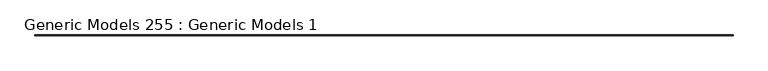
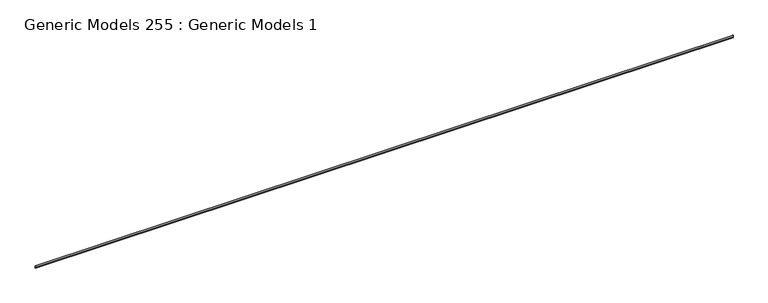
"""IFC4 building model written with IfcOpenShell, lengths in millimetres: proxy geometry, Generic Models 255 : Generic Models 1."""

from ifc_helpers import new_model, si_unit, frame, origin, place, context, project, spatial, polyline, outline, extrude, source, transform, mapped, element, save


def generic_models_255_generic_models_1_b6126c60(model_context):
    return source(origin(), model_context, "Body", "SweptSolid", [
        extrude(outline(polyline([(-29278.6496945, 127648.5865102), (-29298.803311, 127642.1085621), (-29299.6266319, 127637.7365703), (-29300.8746945, 127637.9716019), (-29299.9114994, 127643.0863523), (-29282.7998968, 127648.5865102), (-29300.8746945, 127654.3962666), (-29300.8746945, 127699.3865102), (-29299.6046945, 127699.3865102), (-29299.6046945, 127655.3220459), (-29278.6496945, 127648.5865102)])), frame((-20998.9733045, 0.0, 0.0), z_axis=(1.0, 0.0, 0.0), x_axis=(0.0, 1.0, 0.0)), (0.0, 0.0, 1.0), 19050.0),
    ])


if __name__ == "__main__":
    model = new_model("IFC4")
    model_context = context("Model", 3, world=origin())
    ifc_project = project(units=[si_unit("LENGTHUNIT", "METRE", prefix="MILLI")], contexts=[model_context])
    site = spatial("IfcSite", under=ifc_project)
    building = spatial("IfcBuilding", under=site)
    placement = place(None, origin())
    generic_models_255_generic_models_1_shape = generic_models_255_generic_models_1_b6126c60(model_context)
    element("IfcBuildingElementProxy", 1, Name="Generic Models 255 : Generic Models 1", ObjectType="Generic Models 255 : Generic Models 1", at=placement, inside=building, context=model_context, shape_type="MappedRepresentation", body=[
        mapped(generic_models_255_generic_models_1_shape, transform((0.0, 0.0, 0.0), x_axis=(1.0, 0.0, 0.0), y_axis=(0.0, 1.0, 0.0), z_axis=(0.0, 0.0, 1.0))),
    ])
    save(model, "model.ifc")

# Revit data of these elements
# Element 1 (IfcBuildingElementProxy, "Generic Models 255 : Generic Models 1")
#   Materials on its faces: "_16 GA. COPPER WEEP SCREED W/ MIN. 3 1/2\" ATTACHEMENT FLANGE - LAP UNDERLAYMENT OVER WEED SCREED"
# Materials
#   "_16 GA. COPPER WEEP SCREED W/ MIN. 3 1/2\" ATTACHEMENT FLANGE - LAP UNDERLAYMENT OVER WEED SCREED": class "Generic", colour RGB 253 192 103, transparency 0, Cost = 0
